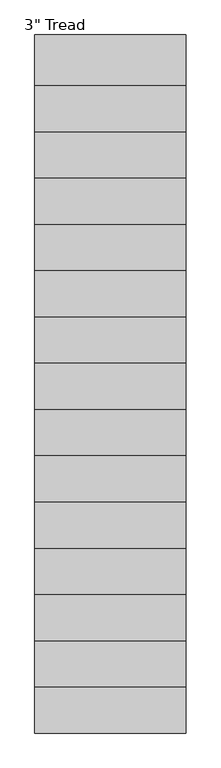
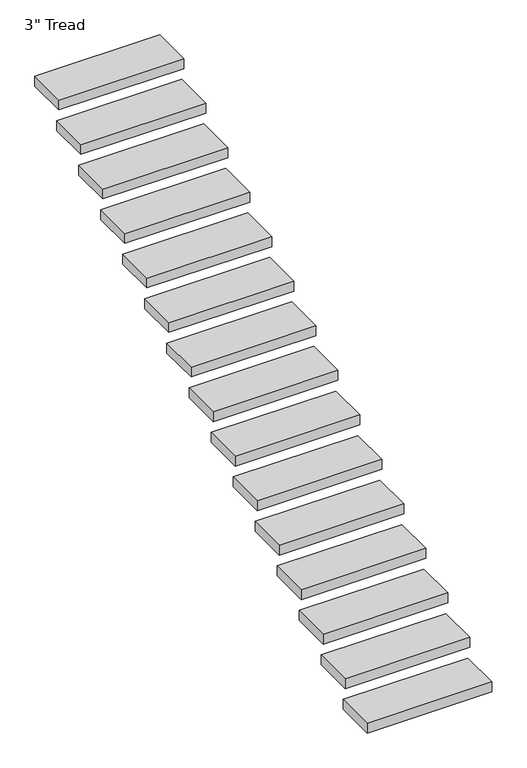
"""IFC4 building model written with IfcOpenShell, lengths in millimetres: stair flight geometry."""

from ifc_helpers import new_model, si_unit, frame, origin, place, context, project, spatial, polyline, outline, extrude, source, transform, mapped, element, save


def stair_flight_a82f31ba(model_context):
    return source(origin(), model_context, "Body", "SweptSolid", [
        extrude(outline(polyline([(32168.5656764, 31238.5118167), (33082.9656764, 31238.5118167), (33082.9656764, 30933.7118167), (32168.5656764, 30933.7118167), (32168.5656764, 31238.5118167)])), frame((0.0, 0.0, 266494.41875), z_axis=(0.0, 0.0, 1.0), x_axis=(1.0, 0.0, 0.0)), (0.0, 0.0, 1.0), 76.2),
        extrude(outline(polyline([(32168.5656764, 31517.9118167), (33082.9656764, 31517.9118167), (33082.9656764, 31213.1118167), (32168.5656764, 31213.1118167), (32168.5656764, 31517.9118167)])), frame((0.0, 0.0, 266669.8375), z_axis=(0.0, 0.0, 1.0), x_axis=(1.0, 0.0, 0.0)), (0.0, 0.0, 1.0), 76.2),
        extrude(outline(polyline([(32168.5656764, 31797.3118167), (33082.9656764, 31797.3118167), (33082.9656764, 31492.5118167), (32168.5656764, 31492.5118167), (32168.5656764, 31797.3118167)])), frame((0.0, 0.0, 266845.25625), z_axis=(0.0, 0.0, 1.0), x_axis=(1.0, 0.0, 0.0)), (0.0, 0.0, 1.0), 76.2),
        extrude(outline(polyline([(32168.5656764, 32076.7118167), (33082.9656764, 32076.7118167), (33082.9656764, 31771.9118167), (32168.5656764, 31771.9118167), (32168.5656764, 32076.7118167)])), frame((0.0, 0.0, 267020.675), z_axis=(0.0, 0.0, 1.0), x_axis=(1.0, 0.0, 0.0)), (0.0, 0.0, 1.0), 76.2),
        extrude(outline(polyline([(32168.5656764, 32356.1118167), (33082.9656764, 32356.1118167), (33082.9656764, 32051.3118167), (32168.5656764, 32051.3118167), (32168.5656764, 32356.1118167)])), frame((0.0, 0.0, 267196.09375), z_axis=(0.0, 0.0, 1.0), x_axis=(1.0, 0.0, 0.0)), (0.0, 0.0, 1.0), 76.2),
        extrude(outline(polyline([(32168.5656764, 32635.5118167), (33082.9656764, 32635.5118167), (33082.9656764, 32330.7118167), (32168.5656764, 32330.7118167), (32168.5656764, 32635.5118167)])), frame((0.0, 0.0, 267371.5125), z_axis=(0.0, 0.0, 1.0), x_axis=(1.0, 0.0, 0.0)), (0.0, 0.0, 1.0), 76.2),
        extrude(outline(polyline([(32168.5656764, 32914.9118167), (33082.9656764, 32914.9118167), (33082.9656764, 32610.1118167), (32168.5656764, 32610.1118167), (32168.5656764, 32914.9118167)])), frame((0.0, 0.0, 267546.93125), z_axis=(0.0, 0.0, 1.0), x_axis=(1.0, 0.0, 0.0)), (0.0, 0.0, 1.0), 76.2),
        extrude(outline(polyline([(32168.5656764, 33194.3118167), (33082.9656764, 33194.3118167), (33082.9656764, 32889.5118167), (32168.5656764, 32889.5118167), (32168.5656764, 33194.3118167)])), frame((0.0, 0.0, 267722.35), z_axis=(0.0, 0.0, 1.0), x_axis=(1.0, 0.0, 0.0)), (0.0, 0.0, 1.0), 76.2),
        extrude(outline(polyline([(32168.5656764, 33473.7118167), (33082.9656764, 33473.7118167), (33082.9656764, 33168.9118167), (32168.5656764, 33168.9118167), (32168.5656764, 33473.7118167)])), frame((0.0, 0.0, 267897.76875), z_axis=(0.0, 0.0, 1.0), x_axis=(1.0, 0.0, 0.0)), (0.0, 0.0, 1.0), 76.2),
        extrude(outline(polyline([(32168.5656764, 33753.1118167), (33082.9656764, 33753.1118167), (33082.9656764, 33448.3118167), (32168.5656764, 33448.3118167), (32168.5656764, 33753.1118167)])), frame((0.0, 0.0, 268073.1875), z_axis=(0.0, 0.0, 1.0), x_axis=(1.0, 0.0, 0.0)), (0.0, 0.0, 1.0), 76.2),
        extrude(outline(polyline([(32168.5656764, 34032.5118167), (33082.9656764, 34032.5118167), (33082.9656764, 33727.7118167), (32168.5656764, 33727.7118167), (32168.5656764, 34032.5118167)])), frame((0.0, 0.0, 268248.60625), z_axis=(0.0, 0.0, 1.0), x_axis=(1.0, 0.0, 0.0)), (0.0, 0.0, 1.0), 76.2),
        extrude(outline(polyline([(32168.5656764, 34311.9118167), (33082.9656764, 34311.9118167), (33082.9656764, 34007.1118167), (32168.5656764, 34007.1118167), (32168.5656764, 34311.9118167)])), frame((0.0, 0.0, 268424.025), z_axis=(0.0, 0.0, 1.0), x_axis=(1.0, 0.0, 0.0)), (0.0, 0.0, 1.0), 76.2),
        extrude(outline(polyline([(32168.5656764, 34591.3118167), (33082.9656764, 34591.3118167), (33082.9656764, 34286.5118167), (32168.5656764, 34286.5118167), (32168.5656764, 34591.3118167)])), frame((0.0, 0.0, 268599.44375), z_axis=(0.0, 0.0, 1.0), x_axis=(1.0, 0.0, 0.0)), (0.0, 0.0, 1.0), 76.2),
        extrude(outline(polyline([(32168.5656764, 34870.7118167), (33082.9656764, 34870.7118167), (33082.9656764, 34565.9118167), (32168.5656764, 34565.9118167), (32168.5656764, 34870.7118167)])), frame((0.0, 0.0, 268774.8625), z_axis=(0.0, 0.0, 1.0), x_axis=(1.0, 0.0, 0.0)), (0.0, 0.0, 1.0), 76.2),
        extrude(outline(polyline([(32168.5656764, 35150.1118167), (33082.9656764, 35150.1118167), (33082.9656764, 34845.3118167), (32168.5656764, 34845.3118167), (32168.5656764, 35150.1118167)])), frame((0.0, 0.0, 268950.28125), z_axis=(0.0, 0.0, 1.0), x_axis=(1.0, 0.0, 0.0)), (0.0, 0.0, 1.0), 76.2),
    ])


if __name__ == "__main__":
    model = new_model("IFC4")
    model_context = context("Model", 3, world=origin())
    ifc_project = project(units=[si_unit("LENGTHUNIT", "METRE", prefix="MILLI")], contexts=[model_context])
    site = spatial("IfcSite", under=ifc_project)
    building = spatial("IfcBuilding", under=site)
    placement = place(None, origin())
    stair_flight_shape = stair_flight_a82f31ba(model_context)
    element("IfcStairFlight", 1, ObjectType="3\" Tread", at=placement, inside=building, context=model_context, shape_type="MappedRepresentation", body=[
        mapped(stair_flight_shape, transform((0.0, 0.0, 0.0), x_axis=(1.0, 0.0, 0.0), y_axis=(0.0, 1.0, 0.0), z_axis=(0.0, 0.0, 1.0))),
    ])
    save(model, "model.ifc")

# Revit data of these elements
# Element 1 (IfcStairFlight, "3\" Tread")
#   Materials on its faces: "GLULAMS BEAMS\n(PRESSURE TREATED W/ PENTA IN SOLVENT) (EXTERIOR STAIN: PENOFIN VERDE EXT. STAIN - COLOR: CEDAR)"
# Materials
#   "GLULAMS BEAMS\n(PRESSURE TREATED W/ PENTA IN SOLVENT) (EXTERIOR STAIN: PENOFIN VERDE EXT. STAIN - COLOR: CEDAR)": class "Wood", colour RGB 164 134 123, transparency 0, Description = "Pinus Echinata", Cost = 0
